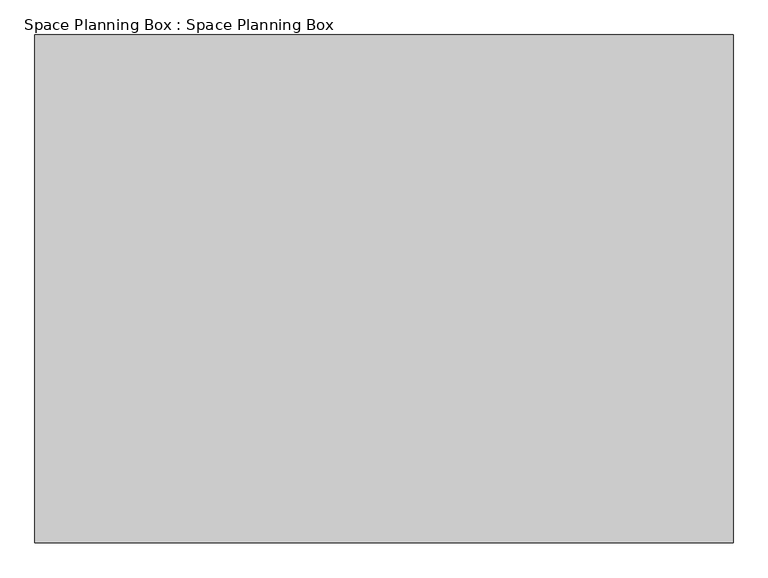
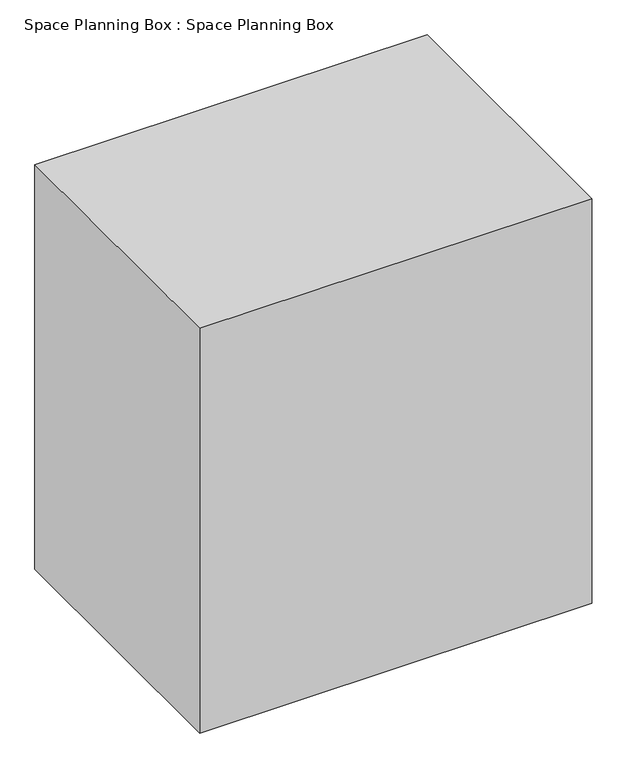
"""IFC4 building model written with IfcOpenShell, lengths in millimetres: proxy geometry, Space Planning Box : Space Planning Box."""

from ifc_helpers import new_model, si_unit, origin, origin_with_axes, place, context, project, spatial, polyline, outline, extrude, source, transform, mapped, element, save


def space_planning_box_space_planning_box_34e84c64(model_context):
    return source(origin(), model_context, "Body", "SweptSolid", [
        extrude(outline(polyline([(2750.0, 2000.0), (2750.0, -2000.0), (-2750.0, -2000.0), (-2750.0, 2000.0), (2750.0, 2000.0)])), origin_with_axes(), (0.0, 0.0, 1.0), 6000.0),
    ])


if __name__ == "__main__":
    model = new_model("IFC4")
    model_context = context("Model", 3, world=origin())
    ifc_project = project(units=[si_unit("LENGTHUNIT", "METRE", prefix="MILLI")], contexts=[model_context])
    site = spatial("IfcSite", under=ifc_project)
    building = spatial("IfcBuilding", under=site)
    placement = place(None, origin())
    space_planning_box_space_planning_box_shape = space_planning_box_space_planning_box_34e84c64(model_context)
    element("IfcBuildingElementProxy", 1, Name="Space Planning Box : Space Planning Box", ObjectType="Space Planning Box : Space Planning Box", at=placement, inside=building, context=model_context, shape_type="MappedRepresentation", body=[
        mapped(space_planning_box_space_planning_box_shape, transform((0.0, 0.0, 0.0), x_axis=(1.0, 0.0, 0.0), y_axis=(0.0, 1.0, 0.0), z_axis=(0.0, 0.0, 1.0))),
    ])
    save(model, "model.ifc")

# Revit data of these elements
# Type "Space Planning Box : Space Planning Box"
#   Type Comments = "..."
#   Room Name [instance default] = "?"
#   Assembly Code = "..."
#   Width [instance default] = 1524 mm
#   Program Area [instance default] = 0 m²
#   Length [instance default] = 1524 mm
#   Height [instance default] = 1524 mm
#   Area [instance default] = 2.32258 m²
#   Fill Color [instance default] = Cyan
#   Default Elevation = 0
# Element 1 (IfcBuildingElementProxy, "Space Planning Box : Space Planning Box")
#   Room Name = "Toilet (M)"
#   Width = 5500 mm
#   Program Area = 72 m²
#   Length = 4000 mm
#   Height = 6000 mm
#   Area = 22 m²
#   Fill Color = Lavender
#   Materials on its faces: "Lavender"
# Materials
#   "Cyan": class "Generic", colour RGB 0 255 255, transparency 0.2, Cost = 0
#   "Lavender": class "Generic", colour RGB 186 85 211, transparency 0.2, Cost = 0
